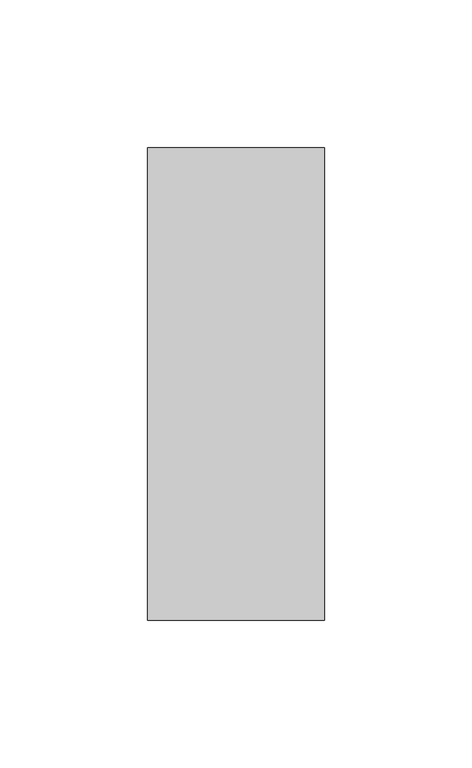
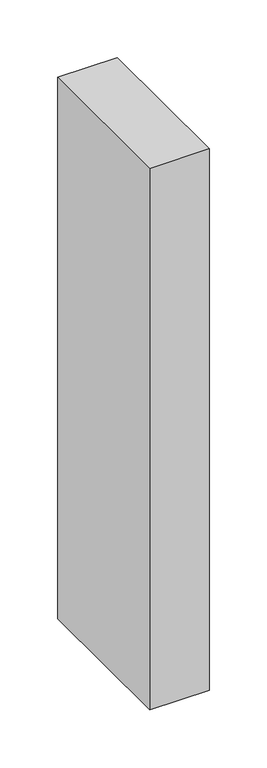
"""IFC4 building model written with IfcOpenShell, lengths in millimetres: column geometry, Madeira de lei-Coluna : Pontalete 6X16cm."""

from ifc_helpers import new_model, si_unit, frame, origin, place, context, project, spatial, polyline, outline, extrude, source, transform, mapped, element, save


def column_df674f92(model_context):
    return source(origin(), model_context, "Body", "SweptSolid", [
        extrude(outline(polyline([(30.0, 80.0), (30.0, -80.0), (-30.0, -80.0), (-30.0, 80.0), (30.0, 80.0)])), frame((0.0, 0.0, 6710.0), z_axis=(0.0, 0.0, 1.0), x_axis=(1.0, 0.0, 0.0)), (0.0, 0.0, 1.0), 575.0),
    ])


if __name__ == "__main__":
    model = new_model("IFC4")
    model_context = context("Model", 3, world=origin())
    ifc_project = project(units=[si_unit("LENGTHUNIT", "METRE", prefix="MILLI")], contexts=[model_context])
    site = spatial("IfcSite", under=ifc_project)
    building = spatial("IfcBuilding", under=site)
    placement = place(None, origin())
    column_shape = column_df674f92(model_context)
    element("IfcColumn", 1, ObjectType="Madeira de lei-Coluna : Pontalete 6X16cm", at=placement, inside=building, context=model_context, shape_type="MappedRepresentation", body=[
        mapped(column_shape, transform((0.0, 0.0, 0.0), x_axis=(1.0, 0.0, 0.0), y_axis=(0.0, 1.0, 0.0), z_axis=(0.0, 0.0, 1.0))),
    ])
    save(model, "model.ifc")

# Revit data of these elements
# Type "Madeira de lei-Coluna : Pontalete 6X16cm"
#   A = 0.01952 m²
#   b = 0.06 m
#   d = 0.16 m
#   Structural Material [instance default] = none
#   Assembly Code = ""
# Element 1 (IfcColumn, "Madeira de lei-Coluna : Pontalete 6X16cm")
#   Structural Material = .MADEIRAMENTO
#   Materials on its faces: ".MADEIRAMENTO"
# Materials
#   ".MADEIRAMENTO": class ".CC_MADEIRAS", colour RGB 212 179 113, transparency 0, Cost = 0
